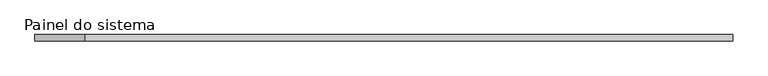
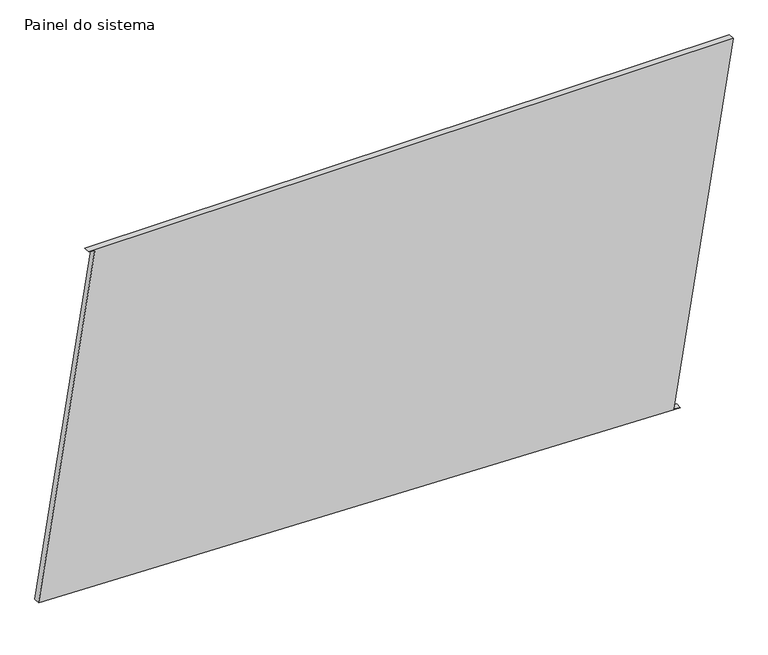
"""IFC4 building model written with IfcOpenShell, lengths in millimetres: plate geometry, Painel do sistema : Envidraçado."""

from ifc_helpers import new_model, si_unit, frame, origin, place, context, project, spatial, polyline, outline, extrude, source, transform, mapped, element, save


def painel_do_sistema_8ff7a025(model_context):
    return source(origin(), model_context, "Body", "SweptSolid", [
        extrude(outline(polyline([(0.0, 1178.140204), (3.9380954, 1153.4523243), (1487.4900209, 1390.101604), (1487.4900209, -1189.7361213), (1483.5519255, -1165.0482416), (72.6946874, -1390.101604), (0.0, 1178.140204)])), frame((0.0, 24.5, 0.0), z_axis=(0.0, 1.0, 0.0), x_axis=(0.0, 0.0, 1.0)), (0.0, 0.0, 1.0), 25.0),
    ])


if __name__ == "__main__":
    model = new_model("IFC4")
    model_context = context("Model", 3, world=origin())
    ifc_project = project(units=[si_unit("LENGTHUNIT", "METRE", prefix="MILLI")], contexts=[model_context])
    site = spatial("IfcSite", under=ifc_project)
    building = spatial("IfcBuilding", under=site)
    placement = place(None, origin())
    painel_do_sistema_shape = painel_do_sistema_8ff7a025(model_context)
    element("IfcPlate", 1, ObjectType="Painel do sistema : Envidraçado", at=placement, inside=building, context=model_context, shape_type="MappedRepresentation", body=[
        mapped(painel_do_sistema_shape, transform((0.0, 0.0, 0.0), x_axis=(1.0, 0.0, 0.0), y_axis=(0.0, 1.0, 0.0), z_axis=(0.0, 0.0, 1.0))),
    ])
    save(model, "model.ifc")

# Revit data of these elements
# Type "Painel do sistema : Envidraçado"
#   Construction Type Id = "GSP4R"
#   Analytic Construction = "Vidraça única Pilkington 1/8 pol"
#   Visual Light Transmittance = 0.9
#   Solar Heat Gain Coefficient = 0.86
#   Heat Transfer Coefficient (U) = 6.7069 W/(m²·K)
# Element 1 (IfcPlate, "Painel do sistema : Envidraçado")
#   Materials on its faces: "Vidro"
# Materials
#   "Vidro": class "Vidro", colour RGB 0 128 192, transparency 0.9, Description = "Vidro de sílica", Cost = 0
